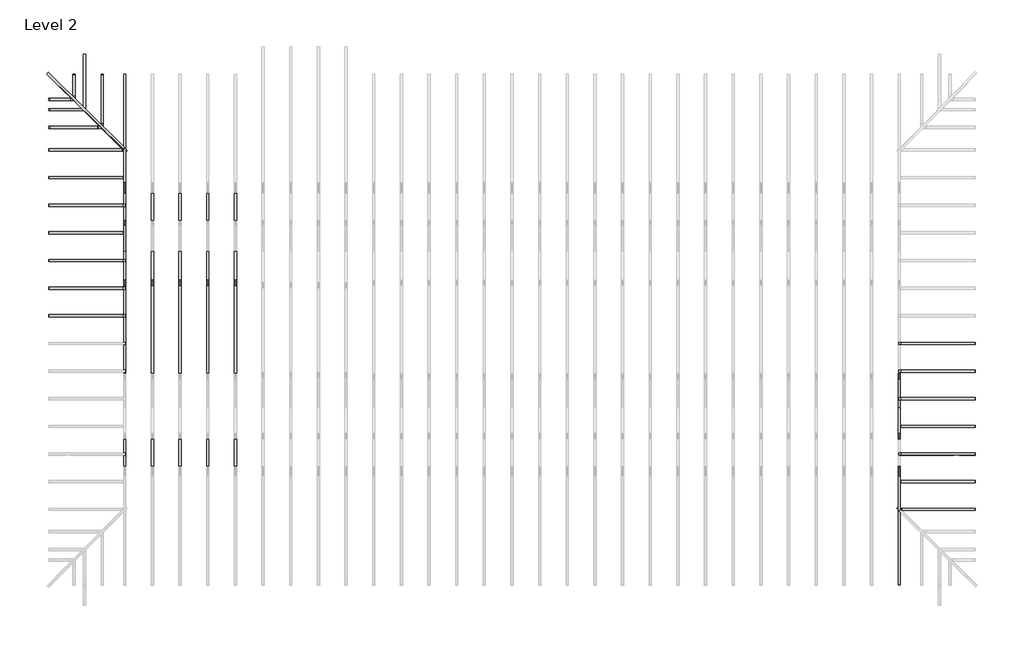
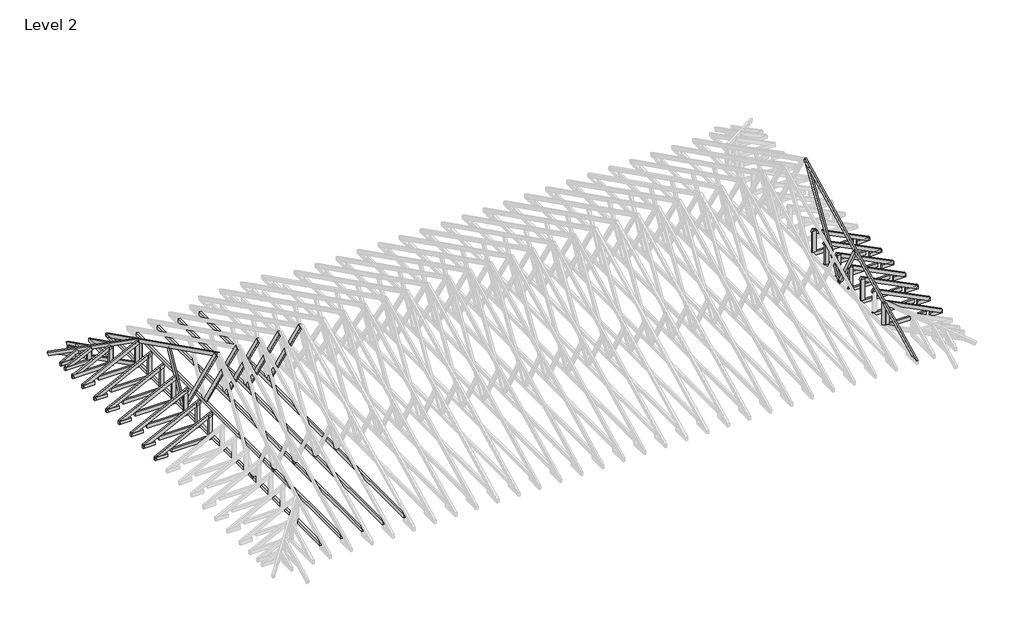
# One storey, part 3 of 5: 93 beams.
"""IFC4 building model written with IfcOpenShell, lengths in millimetres."""

import ifcopenshell
import ifcopenshell.guid

model = None  # the IFC model being written
_history = None  # IfcOwnerHistory: only IFC2X3 demands one
_inside = {}  # id of a spatial element -> (the spatial element, [elements in it])
_under = {}  # id of a project, library or spatial element -> (it, [spatial elements below it])
_declared = {}  # id of a project -> (the project, [libraries it declares])
_typed = {}  # id of a type object -> (the type object, [elements of that type])
_made_of = {}  # id of a material, layer set ... -> (it, [elements and type objects made of it])


def new_model(schema):
    """Start an empty IFC model of exactly this schema.

    Asked for "IFC4X3", IfcOpenShell would pick the latest addendum, in which some entities
    have other attributes; the version numbers below select the first issue.
    IFC2X3 requires an IfcOwnerHistory on every rooted entity: one is made here for all.
    """
    global model, _history
    if schema == "IFC4X3":
        model = ifcopenshell.file(schema_version=(4, 3, 0, 0))
    else:
        model = ifcopenshell.file(schema=schema)
    _inside.clear()
    _under.clear()
    _declared.clear()
    _typed.clear()
    _made_of.clear()
    _history = None
    if model.schema == "IFC2X3":
        org = make("IfcOrganization", Name="unknown")
        user = make(
            "IfcPersonAndOrganization",
            ThePerson=make("IfcPerson", FamilyName="unknown"),
            TheOrganization=org,
        )
        app = make(
            "IfcApplication",
            ApplicationDeveloper=org,
            Version="unknown",
            ApplicationFullName="unknown",
            ApplicationIdentifier="unknown",
        )
        _history = make(
            "IfcOwnerHistory",
            OwningUser=user,
            OwningApplication=app,
            ChangeAction="ADDED",
            CreationDate=0,
        )
    return model


def make(cls, **values):
    """One entity of the class cls with the attributes given. An attribute that is None is left unset."""
    return model.create_entity(
        cls, **{name: value for name, value in values.items() if value is not None}
    )


def rooted(cls, **values):
    """An entity with a GlobalId (a new one), such as an element, a storey or a relation."""
    return make(cls, GlobalId=ifcopenshell.guid.new(), OwnerHistory=_history, **values)


def si_unit(unit_type, name, prefix=None):
    """IfcSIUnit, for example si_unit("LENGTHUNIT", "METRE", prefix="MILLI")."""
    return make("IfcSIUnit", UnitType=unit_type, Prefix=prefix, Name=name)


def assignment(units):
    """IfcUnitAssignment: the units of a project."""
    return None if units is None else make("IfcUnitAssignment", Units=units)


def point(xyz):
    """IfcCartesianPoint."""
    return None if xyz is None else make("IfcCartesianPoint", Coordinates=xyz)


def direction(xyz):
    """IfcDirection."""
    return None if xyz is None else make("IfcDirection", DirectionRatios=xyz)


def frame(location, z_axis=None, x_axis=None):
    """IfcAxis2Placement3D, a coordinate frame: its origin and axes. An axis left out is left unset."""
    return make(
        "IfcAxis2Placement3D",
        Location=point(location),
        Axis=direction(z_axis),
        RefDirection=direction(x_axis),
    )


def origin():
    """The frame at (0, 0, 0) with its axes left unset."""
    return frame((0.0, 0.0, 0.0))


def place(relative_to, where):
    """IfcLocalPlacement: puts the frame where relative to a parent placement (None: the world)."""
    return make(
        "IfcLocalPlacement", PlacementRelTo=relative_to, RelativePlacement=where
    )


def context(
    kind, dimensions, precision=None, world=None, true_north=None, identifier=None
):
    """IfcGeometricRepresentationContext, for example the 3D "Model" context."""
    return make(
        "IfcGeometricRepresentationContext",
        ContextIdentifier=identifier,
        ContextType=kind,
        CoordinateSpaceDimension=dimensions,
        Precision=precision,
        WorldCoordinateSystem=world,
        TrueNorth=true_north,
    )


def project(units=None, contexts=None):
    """IfcProject with its units and contexts."""
    return rooted(
        "IfcProject",
        Name="project",
        RepresentationContexts=contexts,
        UnitsInContext=assignment(units),
    )


def spatial(cls, under=None, at=None, **own):
    """A site, building, storey or space (cls), placed at a placement, below another one or the project."""
    s = rooted(cls, ObjectPlacement=at, **own)
    if under is not None:
        _under.setdefault(under.id(), (under, []))[1].append(s)
    return s


def polyline(points):
    """IfcPolyline through the points."""
    return make("IfcPolyline", Points=[point(p) for p in points])


def outline(outer, holes=None, kind="AREA"):
    """IfcArbitraryClosedProfileDef: a profile drawn as a closed curve; with holes, ...WithVoids."""
    if holes is None:
        return make("IfcArbitraryClosedProfileDef", ProfileType=kind, OuterCurve=outer)
    return make(
        "IfcArbitraryProfileDefWithVoids",
        ProfileType=kind,
        OuterCurve=outer,
        InnerCurves=holes,
    )


def extrude(swept, where, along, depth):
    """IfcExtrudedAreaSolid: the profile swept, set in the frame where, extruded along a direction by depth."""
    return make(
        "IfcExtrudedAreaSolid",
        SweptArea=swept,
        Position=where,
        ExtrudedDirection=direction(along),
        Depth=depth,
    )


def shape(context_of_items, identifier, shape_type, items):
    """IfcShapeRepresentation: the items that make up one representation, for example the "Body"."""
    return make(
        "IfcShapeRepresentation",
        ContextOfItems=context_of_items,
        RepresentationIdentifier=identifier,
        RepresentationType=shape_type,
        Items=items,
    )


def source(mapping_origin, context_of_items, identifier, shape_type, items):
    """IfcRepresentationMap: a shape defined once, which mapped items show again and again."""
    return make(
        "IfcRepresentationMap",
        MappingOrigin=mapping_origin,
        MappedRepresentation=shape(context_of_items, identifier, shape_type, items),
    )


def transform(
    local_origin,
    x_axis=None,
    y_axis=None,
    z_axis=None,
    scale=None,
    scale2=None,
    scale3=None,
    uniform=True,
):
    """IfcCartesianTransformationOperator3D, or its non-uniform kind. x_axis, y_axis, z_axis: its Axis1, 2, 3."""
    if uniform:
        return make(
            "IfcCartesianTransformationOperator3D",
            Axis1=direction(x_axis),
            Axis2=direction(y_axis),
            LocalOrigin=point(local_origin),
            Scale=scale,
            Axis3=direction(z_axis),
        )
    return make(
        "IfcCartesianTransformationOperator3DnonUniform",
        Axis1=direction(x_axis),
        Axis2=direction(y_axis),
        LocalOrigin=point(local_origin),
        Scale=scale,
        Axis3=direction(z_axis),
        Scale2=scale2,
        Scale3=scale3,
    )


def mapped(mapping_source, mapping_target):
    """IfcMappedItem: shows the shape of a source again, moved by a transform."""
    return make(
        "IfcMappedItem", MappingSource=mapping_source, MappingTarget=mapping_target
    )


def made_of(thing, what):
    """Note that an element or type object is made of a material, layer set ...; save() writes the relation."""
    if what is not None:
        _made_of.setdefault(what.id(), (what, []))[1].append(thing)
    return thing


def element(
    cls,
    number,
    at=None,
    inside=None,
    cuts=None,
    type_object=None,
    material=None,
    context=None,
    identifier="Body",
    shape_type=None,
    held_by="IfcProductDefinitionShape",
    body=None,
    shapes=None,
    **own,
):
    """One element of the class cls, such as IfcWall. Its Tag is "e" and its number.

    at: its placement. inside: the storey or other place that contains it. cuts: it is an
    opening in that element (IfcRelVoidsElement). A single representation is given by context,
    identifier, shape_type and body (its items); several are given by shapes. held_by: the class
    of the entity that holds the representations. save() writes the other relations.
    """
    e = rooted(cls, Tag="e%d" % number, ObjectPlacement=at, **own)
    if body is not None:
        shapes = [shape(context, identifier, shape_type, body)]
    if shapes is not None:
        e.Representation = make(held_by, Representations=shapes)
    if inside is not None:
        _inside.setdefault(inside.id(), (inside, []))[1].append(e)
    if cuts is not None:
        rooted(
            "IfcRelVoidsElement", RelatingBuildingElement=cuts, RelatedOpeningElement=e
        )
    if type_object is not None:
        _typed.setdefault(type_object.id(), (type_object, []))[1].append(e)
    return made_of(e, material)


def aggregate(whole, parts):
    """IfcRelAggregates: a whole, such as a stair, and the parts it consists of."""
    return rooted("IfcRelAggregates", RelatingObject=whole, RelatedObjects=parts)


def save(model, path):
    """Write the relations noted so far, then the file.

    IfcRelAggregates (storeys below a building ...), IfcRelContainedInSpatialStructure (elements
    in a storey), IfcRelDefinesByType, IfcRelAssociatesMaterial and IfcRelDeclares: one each for
    every whole, place, type object, material and project.
    """
    for whole, parts in _under.values():
        aggregate(whole, parts)
    for where, things in _inside.values():
        rooted(
            "IfcRelContainedInSpatialStructure",
            RelatedElements=things,
            RelatingStructure=where,
        )
    for kind, things in _typed.values():
        rooted("IfcRelDefinesByType", RelatedObjects=things, RelatingType=kind)
    for what, things in _made_of.values():
        rooted("IfcRelAssociatesMaterial", RelatedObjects=things, RelatingMaterial=what)
    for by, libraries in _declared.values():
        rooted("IfcRelDeclares", RelatingContext=by, RelatedDefinitions=libraries)
    model.write(path)


def beam_90e8f76c(model_context):
    return source(origin(), model_context, "Body", "SweptSolid", [
        extrude(outline(polyline([(307.975, 25.4), (307.975, -25.4), (-47.625, -25.4), (-47.625, 25.4), (307.975, 25.4)])), frame((0.0, 0.0, -50.8), z_axis=(0.0, 0.0, 1.0), x_axis=(1.0, 0.0, 0.0)), (0.0, 0.0, 1.0), 101.6),
    ])


def beam_38027485(model_context):
    return source(origin(), model_context, "Body", "SweptSolid", [
        extrude(outline(polyline([(595.8662636, 25.4), (595.8662636, -25.4), (-609.6, -25.4), (-609.6, 25.4), (595.8662636, 25.4)])), frame((0.0, 0.0, -50.8), z_axis=(0.0, 0.0, 1.0), x_axis=(1.0, 0.0, 0.0)), (0.0, 0.0, 1.0), 101.6),
    ])


def beam_7745fe0f(model_context):
    return source(origin(), model_context, "Body", "SweptSolid", [
        extrude(outline(polyline([(393.7, 25.4), (393.7, -25.4), (-393.7, -25.4), (-393.7, 25.4), (393.7, 25.4)])), frame((0.0, 0.0, -50.8), z_axis=(0.0, 0.0, 1.0), x_axis=(1.0, 0.0, 0.0)), (0.0, 0.0, 1.0), 101.6),
    ])


def beam_85682148(model_context):
    return source(origin(), model_context, "Body", "SweptSolid", [
        extrude(outline(polyline([(595.8662636, -25.4), (-609.6, -25.4), (-609.6, 25.4), (595.8662636, 25.4), (595.8662636, -25.4)])), frame((0.0, 0.0, -50.8), z_axis=(0.0, 0.0, 1.0), x_axis=(1.0, 0.0, 0.0)), (0.0, 0.0, 1.0), 101.6),
    ])


def beam_154fe962(model_context):
    return source(origin(), model_context, "Body", "SweptSolid", [
        extrude(outline(polyline([(228.5999994, 25.4), (228.5999994, -25.4), (-228.6, -25.4), (-228.6, 25.4), (228.5999994, 25.4)])), frame((0.0, 0.0, -50.8), z_axis=(0.0, 0.0, 1.0), x_axis=(1.0, 0.0, 0.0)), (0.0, 0.0, 1.0), 101.6),
    ])


def beam_90eea034(model_context):
    return source(origin(), model_context, "Body", "SweptSolid", [
        extrude(outline(polyline([(821.193698, 25.4), (821.193698, -25.4), (-819.5010489, -25.4), (-819.5010489, 25.4), (821.193698, 25.4)])), frame((0.0, 0.0, -50.8), z_axis=(0.0, 0.0, 1.0), x_axis=(1.0, 0.0, 0.0)), (0.0, 0.0, 1.0), 101.6),
    ])


def beam_a4242642(model_context):
    return source(origin(), model_context, "Body", "SweptSolid", [
        extrude(outline(polyline([(5145.3336481, 25.4), (5145.3336481, -25.4), (-5145.3336481, -25.4), (-5145.3336481, 25.4), (5145.3336481, 25.4)])), frame((0.0, 0.0, -50.8), z_axis=(0.0, 0.0, 1.0), x_axis=(1.0, 0.0, 0.0)), (0.0, 0.0, 1.0), 101.6),
    ])


def beam_16181373(model_context):
    return source(origin(), model_context, "Body", "SweptSolid", [
        extrude(outline(polyline([(819.5010489, 25.4), (819.5010489, -25.4), (-821.193698, -25.4), (-821.193698, 25.4), (819.5010489, 25.4)])), frame((0.0, 0.0, -50.8), z_axis=(0.0, 0.0, 1.0), x_axis=(1.0, 0.0, 0.0)), (0.0, 0.0, 1.0), 101.6),
    ])


def beam_fc8bf4ae(model_context):
    return source(origin(), model_context, "Body", "SweptSolid", [
        extrude(outline(polyline([(1562.6646551, 25.4), (1562.6646551, -25.4), (-1550.1468127, -25.4), (-1550.1468127, 25.4), (1562.6646551, 25.4)])), frame((0.0, 0.0, -50.8), z_axis=(0.0, 0.0, 1.0), x_axis=(1.0, 0.0, 0.0)), (0.0, 0.0, 1.0), 101.6),
    ])


def beam_e838d316(model_context):
    return source(origin(), model_context, "Body", "SweptSolid", [
        extrude(outline(polyline([(1561.1045551, 25.4), (1561.1045551, -25.4), (-1572.5300502, -25.4), (-1572.5300502, 25.4), (1561.1045551, 25.4)])), frame((0.0, 0.0, -50.8), z_axis=(0.0, 0.0, 1.0), x_axis=(1.0, 0.0, 0.0)), (0.0, 0.0, 1.0), 101.6),
    ])


def beam_9afb64f6(model_context):
    return source(origin(), model_context, "Body", "SweptSolid", [
        extrude(outline(polyline([(365.3019367, 25.4), (365.3019367, -25.4), (-314.5019367, -25.4), (-314.5019367, 25.4), (365.3019367, 25.4)])), frame((0.0, 0.0, -50.8), z_axis=(0.0, 0.0, 1.0), x_axis=(1.0, 0.0, 0.0)), (0.0, 0.0, 1.0), 101.6),
    ])


def beam_87710fdd(model_context):
    return source(origin(), model_context, "Body", "SweptSolid", [
        extrude(outline(polyline([(147.1272806, 25.4), (147.1272806, -25.4), (-142.875, -25.4), (-142.875, 25.4), (147.1272806, 25.4)])), frame((0.0, 0.0, -50.8), z_axis=(0.0, 0.0, 1.0), x_axis=(1.0, 0.0, 0.0)), (0.0, 0.0, 1.0), 101.6),
    ])


def beam_29c6d41d(model_context):
    return source(origin(), model_context, "Body", "SweptSolid", [
        extrude(outline(polyline([(350.5042173, 25.4), (350.5042173, -25.4), (-295.4519367, -25.4), (-295.4519367, 25.4), (350.5042173, 25.4)])), frame((0.0, 0.0, -50.8), z_axis=(0.0, 0.0, 1.0), x_axis=(1.0, 0.0, 0.0)), (0.0, 0.0, 1.0), 101.6),
    ])


def beam_af5d22dc(model_context):
    return source(origin(), model_context, "Body", "SweptSolid", [
        extrude(outline(polyline([(571.5, 25.4), (571.5, -25.4), (-609.6, -25.4), (-609.6, 25.4), (571.5, 25.4)])), frame((0.0, 0.0, -50.8), z_axis=(0.0, 0.0, 1.0), x_axis=(1.0, 0.0, 0.0)), (0.0, 0.0, 1.0), 101.6),
    ])


def beam_7b8fa6d1(model_context):
    return source(origin(), model_context, "Body", "SweptSolid", [
        extrude(outline(polyline([(270.7395597, 25.4), (270.7395597, -25.4), (-219.9395597, -25.4), (-219.9395597, 25.4), (270.7395597, 25.4)])), frame((0.0, 0.0, -50.8), z_axis=(0.0, 0.0, 1.0), x_axis=(1.0, 0.0, 0.0)), (0.0, 0.0, 1.0), 101.6),
    ])


def beam_5e172d94(model_context):
    return source(origin(), model_context, "Body", "SweptSolid", [
        extrude(outline(polyline([(595.8662636, 25.4), (595.8662636, -25.4), (-548.2789755, -25.4), (-548.2789755, 25.4), (595.8662636, 25.4)])), frame((0.0, 0.0, -50.8), z_axis=(0.0, 0.0, 1.0), x_axis=(1.0, 0.0, 0.0)), (0.0, 0.0, 1.0), 101.6),
    ])


def beam_42a29ae5(model_context):
    return source(origin(), model_context, "Body", "SweptSolid", [
        extrude(outline(polyline([(270.7395597, -25.4), (-219.9395597, -25.4), (-219.9395597, 25.4), (270.7395597, 25.4), (270.7395597, -25.4)])), frame((0.0, 0.0, -50.8), z_axis=(0.0, 0.0, 1.0), x_axis=(1.0, 0.0, 0.0)), (0.0, 0.0, 1.0), 101.6),
    ])


def beam_11c5b8ca(model_context):
    return source(origin(), model_context, "Body", "SweptSolid", [
        extrude(outline(polyline([(147.1272806, -25.4), (-142.875, -25.4), (-142.875, 25.4), (147.1272806, 25.4), (147.1272806, -25.4)])), frame((0.0, 0.0, -50.8), z_axis=(0.0, 0.0, 1.0), x_axis=(1.0, 0.0, 0.0)), (0.0, 0.0, 1.0), 101.6),
    ])


def beam_5ac0b85f(model_context):
    return source(origin(), model_context, "Body", "SweptSolid", [
        extrude(outline(polyline([(571.5, -25.4), (-584.2, -25.4), (-584.2, 25.4), (571.5, 25.4), (571.5, -25.4)])), frame((0.0, 0.0, -50.8), z_axis=(0.0, 0.0, 1.0), x_axis=(1.0, 0.0, 0.0)), (0.0, 0.0, 1.0), 101.6),
    ])


def beam_99e5442a(model_context):
    return source(origin(), model_context, "Body", "SweptSolid", [
        extrude(outline(polyline([(350.5042173, -25.4), (-295.4519367, -25.4), (-295.4519367, 25.4), (350.5042173, 25.4), (350.5042173, -25.4)])), frame((0.0, 0.0, -50.8), z_axis=(0.0, 0.0, 1.0), x_axis=(1.0, 0.0, 0.0)), (0.0, 0.0, 1.0), 101.6),
    ])


def beam_38e3f9e5(model_context):
    return source(origin(), model_context, "Body", "SweptSolid", [
        extrude(outline(polyline([(595.8662636, -25.4), (-548.2789755, -25.4), (-548.2789755, 25.4), (595.8662636, 25.4), (595.8662636, -25.4)])), frame((0.0, 0.0, -50.8), z_axis=(0.0, 0.0, 1.0), x_axis=(1.0, 0.0, 0.0)), (0.0, 0.0, 1.0), 101.6),
    ])


def beam_7aad778a(model_context):
    return source(origin(), model_context, "Body", "SweptSolid", [
        extrude(outline(polyline([(307.975, -25.4), (-47.625, -25.4), (-47.625, 25.4), (307.975, 25.4), (307.975, -25.4)])), frame((0.0, 0.0, -50.8), z_axis=(0.0, 0.0, 1.0), x_axis=(1.0, 0.0, 0.0)), (0.0, 0.0, 1.0), 101.6),
    ])


def beam_878446a4(model_context):
    return source(origin(), model_context, "Body", "SweptSolid", [
        extrude(outline(polyline([(63.8057136, 25.4), (63.8057136, -25.4), (-59.553433, -25.4), (-59.553433, 25.4), (63.8057136, 25.4)])), frame((0.0, 0.0, -50.8), z_axis=(0.0, 0.0, 1.0), x_axis=(1.0, 0.0, 0.0)), (0.0, 0.0, 1.0), 101.6),
    ])


def beam_bc99fd75(model_context):
    return source(origin(), model_context, "Body", "SweptSolid", [
        extrude(outline(polyline([(222.3387319, 25.4), (222.3387319, -25.4), (-231.775, -25.4), (-231.775, 25.4), (222.3387319, 25.4)])), frame((0.0, 0.0, -50.8), z_axis=(0.0, 0.0, 1.0), x_axis=(1.0, 0.0, 0.0)), (0.0, 0.0, 1.0), 101.6),
    ])


def beam_efe25585(model_context):
    return source(origin(), model_context, "Body", "SweptSolid", [
        extrude(outline(polyline([(222.3387319, -25.4), (-231.775, -25.4), (-231.775, 25.4), (222.3387319, 25.4), (222.3387319, -25.4)])), frame((0.0, 0.0, -50.8), z_axis=(0.0, 0.0, 1.0), x_axis=(1.0, 0.0, 0.0)), (0.0, 0.0, 1.0), 101.6),
    ])


def beam_dfed05dc(model_context):
    return source(origin(), model_context, "Body", "SweptSolid", [
        extrude(outline(polyline([(63.8057136, -25.4), (-59.553433, -25.4), (-59.553433, 25.4), (63.8057136, 25.4), (63.8057136, -25.4)])), frame((0.0, 0.0, -50.8), z_axis=(0.0, 0.0, 1.0), x_axis=(1.0, 0.0, 0.0)), (0.0, 0.0, 1.0), 101.6),
    ])


def beam_b8261971(model_context):
    return source(origin(), model_context, "Body", "SweptSolid", [
        extrude(outline(polyline([(233.4866591, 25.4), (233.4866591, -25.4), (-1841.8619641, -25.4), (-1841.8619641, 25.4), (233.4866591, 25.4)])), frame((0.0, 0.0, -50.8), z_axis=(0.0, 0.0, 1.0), x_axis=(1.0, 0.0, 0.0)), (0.0, 0.0, 1.0), 101.6),
    ])


def beam_925b2549(model_context):
    return source(origin(), model_context, "Body", "SweptSolid", [
        extrude(outline(polyline([(371.7582386, -25.4), (-368.3, -25.4), (-368.3, 25.4), (371.7582386, 25.4), (371.7582386, -25.4)])), frame((0.0, 0.0, -50.8), z_axis=(0.0, 0.0, 1.0), x_axis=(1.0, 0.0, 0.0)), (0.0, 0.0, 1.0), 101.6),
    ])


model = new_model("IFC4")

# Units and contexts
model_context = context("Model", 3, world=origin())
ifc_project = project(units=[si_unit("LENGTHUNIT", "METRE", prefix="MILLI")], contexts=[model_context])

# Site, building, storey
site = spatial("IfcSite", under=ifc_project)
building = spatial("IfcBuilding", under=site)
storey = spatial("IfcBuildingStorey", under=building, Name="Level 2", Elevation=2768.6)

# Beams
placement = place(None, origin())
element("IfcBeam", 1, ObjectType="Dimension Lumber : BLDG 6241 2X4\" TRUSS MEMBER", at=placement, inside=storey, context=model_context, shape_type="SweptSolid", body=[
    extrude(outline(polyline([(0.0, -50.8), (0.0, 0.0), (6302.2496334, 0.0), (6302.2496334, -50.8), (0.0, -50.8)])), frame((-16607.414829, -17.2791662, 5496.1115355), z_axis=(0.0, 0.447213595499958, 0.894427190999916), x_axis=(0.0, 0.894427190999916, -0.447213595499958)), (0.0, 0.0, 1.0), 101.6),
])
element("IfcBeam", 2, ObjectType="Dimension Lumber : BLDG 6241 2X4\" TRUSS MEMBER", at=placement, inside=storey, context=model_context, shape_type="SweptSolid", body=[
    extrude(outline(polyline([(0.0, -50.8), (0.0, 0.0), (1828.8, 0.0), (1828.8, -50.8), (0.0, -50.8)])), frame((-18206.2149687, 3404.3284114, 2681.1076769), z_axis=(-0.44721359549995937, 0.0, 0.8944271909999152), x_axis=(0.8944271909999152, 0.0, 0.44721359549995937)), (0.0, 0.0, 1.0), 101.6),
])
element("IfcBeam", 3, ObjectType="Dimension Lumber : BLDG 6241 2X4\" TRUSS MEMBER", at=placement, inside=storey, context=model_context, shape_type="SweptSolid", body=[
    extrude(outline(polyline([(1e-07, -50.8), (0.0, 0.0), (2518.7475141, 0.0), (2518.7475141, -50.8), (1e-07, -50.8)])), frame((-16592.3107327, 3976.1580779, 3516.9362486), z_axis=(-0.2218309319850432, 0.2532052771584921, 0.9416358772018717), x_axis=(-0.6716162760239249, 0.6604274920267121, -0.33580813801196385)), (0.0, 0.0, 1.0), 101.6),
])
element("IfcBeam", 4, ObjectType="Dimension Lumber : BLDG 6241 2X4\" TRUSS MEMBER", at=placement, inside=storey, context=model_context, shape_type="SweptSolid", body=[
    extrude(outline(polyline([(0.0, -50.8), (0.0, 0.0), (1203.6219076, 0.0), (1203.6219076, -50.8), (0.0, -50.8)])), frame((-18207.7449824, 4509.2284114, 2680.3426701), z_axis=(-0.44721359549995937, 0.0, 0.8944271909999152), x_axis=(0.8944271909999152, 0.0, 0.44721359549995937)), (0.0, 0.0, 1.0), 101.6),
])
element("IfcBeam", 5, ObjectType="Dimension Lumber : BLDG 6241 2X4\" TRUSS MEMBER", at=placement, inside=storey, context=model_context, shape_type="SweptSolid", body=[
    extrude(outline(polyline([(0.0, -50.8), (0.0, 0.0), (844.55, 0.0), (844.55, -50.8), (0.0, -50.8)])), frame((-18212.4885612, 4902.9284114, 2677.9708807), z_axis=(-0.4472135954999599, 0.0, 0.894427190999915), x_axis=(0.894427190999915, 0.0, 0.4472135954999599)), (0.0, 0.0, 1.0), 101.6),
])
element("IfcBeam", 6, ObjectType="Dimension Lumber : BLDG 6241 2X4\" TRUSS MEMBER", at=placement, inside=storey, context=model_context, shape_type="SweptSolid", body=[
    extrude(outline(polyline([(0.0, -50.8), (0.0, 0.0), (6302.3539791, 0.0), (6302.3539791, -50.8), (0.0, -50.8)])), frame((461.385171, -5565.5155384, 2678.5857718), z_axis=(0.0, -0.447213595499958, 0.894427190999916), x_axis=(0.0, 0.894427190999916, 0.447213595499958)), (0.0, 0.0, 1.0), 101.6),
])
element("IfcBeam", 7, ObjectType="Dimension Lumber : BLDG 6241 2X4\" TRUSS MEMBER", at=placement, inside=storey, context=model_context, shape_type="SweptSolid", body=[
    extrude(outline(polyline([(0.0, -50.8), (0.0, 0.0), (1787.5128974, 0.0), (1787.5128974, -50.8), (0.0, -50.8)])), frame((-18206.2149687, 4013.9284114, 2681.1076769), z_axis=(-0.44721359549995937, 0.0, 0.8944271909999152), x_axis=(0.8944271909999152, 0.0, 0.44721359549995937)), (0.0, 0.0, 1.0), 101.6),
])
element("IfcBeam", 8, ObjectType="Dimension Lumber : BLDG 6241 2X4\" TRUSS MEMBER", at=placement, inside=storey, context=model_context, shape_type="SweptSolid", body=[
    extrude(outline(polyline([(0.0, -50.8), (0.0, 0.0), (1828.8, 0.0), (1828.8, -50.8), (0.0, -50.8)])), frame((-18206.2149687, 2794.7284114, 2681.1076769), z_axis=(-0.44721359549995937, 0.0, 0.8944271909999152), x_axis=(0.8944271909999152, 0.0, 0.44721359549995937)), (0.0, 0.0, 1.0), 101.6),
])
element("IfcBeam", 9, ObjectType="Dimension Lumber : BLDG 6241 2X4\" TRUSS MEMBER", at=placement, inside=storey, context=model_context, shape_type="SweptSolid", body=[
    extrude(outline(polyline([(0.0, -50.8), (0.0, 0.0), (1828.8, 0.0), (1828.8, -50.8), (0.0, -50.8)])), frame((-18206.2149687, 2185.1284114, 2681.1076769), z_axis=(-0.44721359549995937, 0.0, 0.8944271909999152), x_axis=(0.8944271909999152, 0.0, 0.44721359549995937)), (0.0, 0.0, 1.0), 101.6),
])
element("IfcBeam", 10, ObjectType="Dimension Lumber : BLDG 6241 2X4\" TRUSS MEMBER", at=placement, inside=storey, context=model_context, shape_type="SweptSolid", body=[
    extrude(outline(polyline([(0.0, -50.8), (0.0, 0.0), (1828.8, 0.0), (1828.8, -50.8), (0.0, -50.8)])), frame((-18206.2149687, 1575.5284114, 2681.1076769), z_axis=(-0.44721359549995937, 0.0, 0.8944271909999152), x_axis=(0.8944271909999152, 0.0, 0.44721359549995937)), (0.0, 0.0, 1.0), 101.6),
])
element("IfcBeam", 11, ObjectType="Dimension Lumber : BLDG 6241 2X4\" TRUSS MEMBER", at=placement, inside=storey, context=model_context, shape_type="SweptSolid", body=[
    extrude(outline(polyline([(0.0, -50.8), (0.0, 0.0), (1828.8, 0.0), (1828.8, -50.8), (0.0, -50.8)])), frame((-18206.2149687, 965.9284114, 2681.1076769), z_axis=(-0.44721359549995937, 0.0, 0.8944271909999152), x_axis=(0.8944271909999152, 0.0, 0.44721359549995937)), (0.0, 0.0, 1.0), 101.6),
])
element("IfcBeam", 12, ObjectType="Dimension Lumber : BLDG 6241 2X4\" TRUSS MEMBER", at=placement, inside=storey, context=model_context, shape_type="SweptSolid", body=[
    extrude(outline(polyline([(0.0, -50.8), (0.0, 0.0), (1828.8, 0.0), (1828.8, -50.8), (0.0, -50.8)])), frame((-18206.2149687, 356.3284114, 2681.1076769), z_axis=(-0.44721359549995937, 0.0, 0.8944271909999152), x_axis=(0.8944271909999152, 0.0, 0.44721359549995937)), (0.0, 0.0, 1.0), 101.6),
])
element("IfcBeam", 13, ObjectType="Dimension Lumber : BLDG 6241 2X4\" TRUSS MEMBER", at=placement, inside=storey, context=model_context, shape_type="SweptSolid", body=[
    extrude(outline(polyline([(0.0, 50.8), (1203.6219076, 50.8), (1203.6219076, 0.0), (0.0, 0.0), (0.0, 50.8)])), frame((-17102.714829, 5614.2585647, 2680.3426701), z_axis=(0.0, 0.44721359549995937, 0.8944271909999152), x_axis=(0.0, -0.8944271909999152, 0.44721359549995937)), (0.0, 0.0, 1.0), 101.6),
])
element("IfcBeam", 14, ObjectType="Dimension Lumber : BLDG 6241 2X4\" TRUSS MEMBER", at=placement, inside=storey, context=model_context, shape_type="SweptSolid", body=[
    extrude(outline(polyline([(0.0, 50.8), (1334.5727744, 50.8), (1334.5727744, 0.0), (0.0, 0.0), (0.0, 50.8)])), frame((-17496.414829, 6057.2918371, 2458.8260339), z_axis=(0.0, 0.4472135954999599, 0.894427190999915), x_axis=(0.0, -0.894427190999915, 0.4472135954999599)), (0.0, 0.0, 1.0), 101.6),
])
element("IfcBeam", 15, ObjectType="Dimension Lumber : BLDG 6241 2X4\" TRUSS MEMBER", at=placement, inside=storey, context=model_context, shape_type="SweptSolid", body=[
    extrude(outline(polyline([(0.0, 50.8), (1828.8, 50.8), (1828.8, 0.0), (0.0, 0.0), (0.0, 50.8)])), frame((2110.9853106, -253.2715886, 2681.1076769), z_axis=(0.44721359549995937, 0.0, 0.8944271909999152), x_axis=(-0.8944271909999152, 0.0, 0.44721359549995937)), (0.0, 0.0, 1.0), 101.6),
])
element("IfcBeam", 16, ObjectType="Dimension Lumber : BLDG 6241 2X4\" TRUSS MEMBER", at=placement, inside=storey, context=model_context, shape_type="SweptSolid", body=[
    extrude(outline(polyline([(0.0, 50.8), (1828.8, 50.8), (1828.8, 0.0), (0.0, 0.0), (0.0, 50.8)])), frame((2110.9853106, -862.8715886, 2681.1076769), z_axis=(0.44721359549995937, 0.0, 0.8944271909999152), x_axis=(-0.8944271909999152, 0.0, 0.44721359549995937)), (0.0, 0.0, 1.0), 101.6),
])
element("IfcBeam", 17, ObjectType="Dimension Lumber : BLDG 6241 2X4\" TRUSS MEMBER", at=placement, inside=storey, context=model_context, shape_type="SweptSolid", body=[
    extrude(outline(polyline([(0.0, 50.8), (1828.8, 50.8), (1828.8, 0.0), (0.0, 0.0), (0.0, 50.8)])), frame((2110.9853106, -1472.4715886, 2681.1076769), z_axis=(0.44721359549995937, 0.0, 0.8944271909999152), x_axis=(-0.8944271909999152, 0.0, 0.44721359549995937)), (0.0, 0.0, 1.0), 101.6),
])
element("IfcBeam", 18, ObjectType="Dimension Lumber : BLDG 6241 2X4\" TRUSS MEMBER", at=placement, inside=storey, context=model_context, shape_type="SweptSolid", body=[
    extrude(outline(polyline([(0.0, 50.8), (1828.8, 50.8), (1828.8, 0.0), (0.0, 0.0), (0.0, 50.8)])), frame((2110.9853106, -2082.0715886, 2681.1076769), z_axis=(0.44721359549995937, 0.0, 0.8944271909999152), x_axis=(-0.8944271909999152, 0.0, 0.44721359549995937)), (0.0, 0.0, 1.0), 101.6),
])
element("IfcBeam", 19, ObjectType="Dimension Lumber : BLDG 6241 2X4\" TRUSS MEMBER", at=placement, inside=storey, context=model_context, shape_type="SweptSolid", body=[
    extrude(outline(polyline([(0.0, 50.8), (1828.8, 50.8), (1828.8, 0.0), (0.0, 0.0), (0.0, 50.8)])), frame((2110.9853106, -2691.6715886, 2681.1076769), z_axis=(0.44721359549995937, 0.0, 0.8944271909999152), x_axis=(-0.8944271909999152, 0.0, 0.44721359549995937)), (0.0, 0.0, 1.0), 101.6),
])
element("IfcBeam", 20, ObjectType="Dimension Lumber : BLDG 6241 2X4\" TRUSS MEMBER", at=placement, inside=storey, context=model_context, shape_type="SweptSolid", body=[
    extrude(outline(polyline([(0.0, 50.8), (1828.8, 50.8), (1828.8, 0.0), (0.0, 0.0), (0.0, 50.8)])), frame((2110.9853106, -3301.2715886, 2681.1076769), z_axis=(0.44721359549995937, 0.0, 0.8944271909999152), x_axis=(-0.8944271909999152, 0.0, 0.44721359549995937)), (0.0, 0.0, 1.0), 101.6),
])
element("IfcBeam", 21, ObjectType="Dimension Lumber : BLDG 6241 2X4\" TRUSS MEMBER", at=placement, inside=storey, context=model_context, shape_type="SweptSolid", body=[
    extrude(outline(polyline([(0.0, 50.8), (1787.5128973, 50.8), (1787.5128973, 0.0), (0.0, 0.0), (0.0, 50.8)])), frame((2110.9853106, -3910.8715886, 2681.1076769), z_axis=(0.44721359549995937, 0.0, 0.8944271909999152), x_axis=(-0.8944271909999152, 0.0, 0.44721359549995937)), (0.0, 0.0, 1.0), 101.6),
])
element("IfcBeam", 22, ObjectType="Dimension Lumber : BLDG 6241 2X4\" TRUSS MEMBER", at=placement, inside=storey, context=model_context, shape_type="SweptSolid", body=[
    extrude(outline(polyline([(0.0, -50.8), (0.0, 0.0), (546.1, 0.0), (546.1, -50.8), (0.0, -50.8)])), frame((-18212.1757804, 5131.5284114, 2678.127271), z_axis=(-0.4472135954999593, 0.0, 0.8944271909999153), x_axis=(0.8944271909999153, 0.0, 0.4472135954999593)), (0.0, 0.0, 1.0), 101.6),
])
element("IfcBeam", 23, ObjectType="Dimension Lumber : BLDG 6241 2X4\" TRUSS MEMBER", at=placement, inside=storey, context=model_context, shape_type="SweptSolid", body=[
    extrude(outline(polyline([(0.0, 50.8), (546.1, 50.8), (546.1, 0.0), (0.0, 0.0), (0.0, 50.8)])), frame((-17725.014829, 5618.6893628, 2678.127271), z_axis=(0.0, 0.4472135954999592, 0.8944271909999153), x_axis=(0.0, -0.8944271909999153, 0.4472135954999592)), (0.0, 0.0, 1.0), 101.6),
])
beam_shape = beam_90e8f76c(model_context)
element("IfcBeam", 24, ObjectType="Dimension Lumber : BLDG 6241 2X4\" TRUSS MEMBER", at=placement, inside=storey, context=model_context, shape_type="MappedRepresentation", body=[
    mapped(beam_shape, transform((-18210.789829, 3378.9284114, 2717.8), x_axis=(1.0, 0.0, 0.0), y_axis=(0.0, 1.0, 0.0), z_axis=(0.0, 0.0, 1.0))),
])
element("IfcBeam", 25, ObjectType="Dimension Lumber : BLDG 6241 2X4\" TRUSS MEMBER", at=placement, inside=storey, context=model_context, shape_type="MappedRepresentation", body=[
    mapped(beam_shape, transform((-18210.789829, 3988.5284114, 2717.8), x_axis=(1.0, 0.0, 0.0), y_axis=(0.0, 1.0, 0.0), z_axis=(0.0, 0.0, 1.0))),
])
element("IfcBeam", 26, ObjectType="Dimension Lumber : BLDG 6241 2X4\" TRUSS MEMBER", at=placement, inside=storey, context=model_context, shape_type="MappedRepresentation", body=[
    mapped(beam_shape, transform((-18210.789829, 2769.3284114, 2717.8), x_axis=(1.0, 0.0, 0.0), y_axis=(0.0, 1.0, 0.0), z_axis=(0.0, 0.0, 1.0))),
])
element("IfcBeam", 27, ObjectType="Dimension Lumber : BLDG 6241 2X4\" TRUSS MEMBER", at=placement, inside=storey, context=model_context, shape_type="MappedRepresentation", body=[
    mapped(beam_shape, transform((-18210.789829, 2159.7284114, 2717.8), x_axis=(1.0, 0.0, 0.0), y_axis=(0.0, 1.0, 0.0), z_axis=(0.0, 0.0, 1.0))),
])
element("IfcBeam", 28, ObjectType="Dimension Lumber : BLDG 6241 2X4\" TRUSS MEMBER", at=placement, inside=storey, context=model_context, shape_type="MappedRepresentation", body=[
    mapped(beam_shape, transform((-18210.789829, 1550.1284114, 2717.8), x_axis=(1.0, 0.0, 0.0), y_axis=(0.0, 1.0, 0.0), z_axis=(0.0, 0.0, 1.0))),
])
element("IfcBeam", 29, ObjectType="Dimension Lumber : BLDG 6241 2X4\" TRUSS MEMBER", at=placement, inside=storey, context=model_context, shape_type="MappedRepresentation", body=[
    mapped(beam_shape, transform((-18210.789829, 940.5284114, 2717.8), x_axis=(1.0, 0.0, 0.0), y_axis=(0.0, 1.0, 0.0), z_axis=(0.0, 0.0, 1.0))),
])
element("IfcBeam", 30, ObjectType="Dimension Lumber : BLDG 6241 2X4\" TRUSS MEMBER", at=placement, inside=storey, context=model_context, shape_type="MappedRepresentation", body=[
    mapped(beam_shape, transform((-18210.789829, 330.9284114, 2717.8), x_axis=(1.0, 0.0, 0.0), y_axis=(0.0, 1.0, 0.0), z_axis=(0.0, 0.0, 1.0))),
])
beam_2_shape = beam_38027485(model_context)
element("IfcBeam", 31, ObjectType="Dimension Lumber : BLDG 6241 2X4\" TRUSS MEMBER", at=placement, inside=storey, context=model_context, shape_type="MappedRepresentation", body=[
    mapped(beam_2_shape, transform((-17191.614829, 3378.9284114, 2819.4), x_axis=(-1.0, 0.0, 0.0), y_axis=(0.0, -1.0, 0.0), z_axis=(0.0, 0.0, 1.0))),
])
element("IfcBeam", 32, ObjectType="Dimension Lumber : BLDG 6241 2X4\" TRUSS MEMBER", at=placement, inside=storey, context=model_context, shape_type="MappedRepresentation", body=[
    mapped(beam_2_shape, transform((-17191.614829, 2769.3284114, 2819.4), x_axis=(-1.0, 0.0, 0.0), y_axis=(0.0, -1.0, 0.0), z_axis=(0.0, 0.0, 1.0))),
])
element("IfcBeam", 33, ObjectType="Dimension Lumber : BLDG 6241 2X4\" TRUSS MEMBER", at=placement, inside=storey, context=model_context, shape_type="MappedRepresentation", body=[
    mapped(beam_2_shape, transform((-17191.614829, 2159.7284114, 2819.4), x_axis=(-1.0, 0.0, 0.0), y_axis=(0.0, -1.0, 0.0), z_axis=(0.0, 0.0, 1.0))),
])
element("IfcBeam", 34, ObjectType="Dimension Lumber : BLDG 6241 2X4\" TRUSS MEMBER", at=placement, inside=storey, context=model_context, shape_type="MappedRepresentation", body=[
    mapped(beam_2_shape, transform((-17191.614829, 1550.1284114, 2819.4), x_axis=(-1.0, 0.0, 0.0), y_axis=(0.0, -1.0, 0.0), z_axis=(0.0, 0.0, 1.0))),
])
element("IfcBeam", 35, ObjectType="Dimension Lumber : BLDG 6241 2X4\" TRUSS MEMBER", at=placement, inside=storey, context=model_context, shape_type="MappedRepresentation", body=[
    mapped(beam_2_shape, transform((-17191.614829, 940.5284114, 2819.4), x_axis=(-1.0, 0.0, 0.0), y_axis=(0.0, -1.0, 0.0), z_axis=(0.0, 0.0, 1.0))),
])
element("IfcBeam", 36, ObjectType="Dimension Lumber : BLDG 6241 2X4\" TRUSS MEMBER", at=placement, inside=storey, context=model_context, shape_type="MappedRepresentation", body=[
    mapped(beam_2_shape, transform((-17191.614829, 330.9284114, 2819.4), x_axis=(-1.0, 0.0, 0.0), y_axis=(0.0, -1.0, 0.0), z_axis=(0.0, 0.0, 1.0))),
])
beam_3_shape = beam_7745fe0f(model_context)
element("IfcBeam", 37, ObjectType="Dimension Lumber : BLDG 6241 2X4\" TRUSS MEMBER", at=placement, inside=storey, context=model_context, shape_type="MappedRepresentation", body=[
    mapped(beam_3_shape, transform((-17864.714829, 4877.5284114, 2728.7708807), x_axis=(-1.0, 0.0, 0.0), y_axis=(0.0, -1.0, 0.0), z_axis=(0.0, 0.0, 1.0))),
])
beam_4_shape = beam_85682148(model_context)
element("IfcBeam", 38, ObjectType="Dimension Lumber : BLDG 6241 2X4\" TRUSS MEMBER", at=placement, inside=storey, context=model_context, shape_type="MappedRepresentation", body=[
    mapped(beam_4_shape, transform((1096.385171, -278.6715886, 2819.4), x_axis=(1.0, 0.0, 0.0), y_axis=(0.0, 1.0, 0.0), z_axis=(0.0, 0.0, 1.0))),
])
element("IfcBeam", 39, ObjectType="Dimension Lumber : BLDG 6241 2X4\" TRUSS MEMBER", at=placement, inside=storey, context=model_context, shape_type="MappedRepresentation", body=[
    mapped(beam_4_shape, transform((1096.385171, -888.2715886, 2819.4), x_axis=(1.0, 0.0, 0.0), y_axis=(0.0, 1.0, 0.0), z_axis=(0.0, 0.0, 1.0))),
])
element("IfcBeam", 40, ObjectType="Dimension Lumber : BLDG 6241 2X4\" TRUSS MEMBER", at=placement, inside=storey, context=model_context, shape_type="MappedRepresentation", body=[
    mapped(beam_4_shape, transform((1096.385171, -1497.8715886, 2819.4), x_axis=(1.0, 0.0, 0.0), y_axis=(0.0, 1.0, 0.0), z_axis=(0.0, 0.0, 1.0))),
])
element("IfcBeam", 41, ObjectType="Dimension Lumber : BLDG 6241 2X4\" TRUSS MEMBER", at=placement, inside=storey, context=model_context, shape_type="MappedRepresentation", body=[
    mapped(beam_4_shape, transform((1096.385171, -2107.4715886, 2819.4), x_axis=(1.0, 0.0, 0.0), y_axis=(0.0, 1.0, 0.0), z_axis=(0.0, 0.0, 1.0))),
])
element("IfcBeam", 42, ObjectType="Dimension Lumber : BLDG 6241 2X4\" TRUSS MEMBER", at=placement, inside=storey, context=model_context, shape_type="MappedRepresentation", body=[
    mapped(beam_4_shape, transform((1096.385171, -2717.0715886, 2819.4), x_axis=(1.0, 0.0, 0.0), y_axis=(0.0, 1.0, 0.0), z_axis=(0.0, 0.0, 1.0))),
])
element("IfcBeam", 43, ObjectType="Dimension Lumber : BLDG 6241 2X4\" TRUSS MEMBER", at=placement, inside=storey, context=model_context, shape_type="MappedRepresentation", body=[
    mapped(beam_4_shape, transform((1096.385171, -3326.6715886, 2819.4), x_axis=(1.0, 0.0, 0.0), y_axis=(0.0, 1.0, 0.0), z_axis=(0.0, 0.0, 1.0))),
])
beam_5_shape = beam_154fe962(model_context)
element("IfcBeam", 44, ObjectType="Dimension Lumber : BLDG 6241 2X4\" TRUSS MEMBER", at=placement, inside=storey, context=model_context, shape_type="MappedRepresentation", body=[
    mapped(beam_5_shape, transform((-16582.014829, 5436.3284114, 2717.8), x_axis=(0.0, -1.0, 0.0), y_axis=(1.0, 0.0, 0.0), z_axis=(0.0, 0.0, 1.0))),
])
beam_6_shape = beam_90eea034(model_context)
element("IfcBeam", 45, ObjectType="Dimension Lumber : BLDG 6241 2X4\" TRUSS MEMBER", at=placement, inside=storey, context=model_context, shape_type="MappedRepresentation", body=[
    mapped(beam_6_shape, transform((-16582.014829, 2147.8781861, 3552.5770493), x_axis=(0.0, -0.4803172630852001, -0.8770948220017848), y_axis=(-1.0, 0.0, 0.0), z_axis=(0.0, 0.8770948220017848, -0.4803172630852001))),
])
beam_7_shape = beam_a4242642(model_context)
element("IfcBeam", 46, ObjectType="Dimension Lumber : BLDG 6241 2X4\" TRUSS MEMBER", at=placement, inside=storey, context=model_context, shape_type="MappedRepresentation", body=[
    mapped(beam_7_shape, transform((-16582.014829, 26.1284114, 2819.4), x_axis=(0.0, -1.0, 0.0), y_axis=(1.0, 0.0, 0.0), z_axis=(0.0, 0.0, 1.0))),
])
element("IfcBeam", 47, ObjectType="Dimension Lumber : BLDG 6241 2X4\" TRUSS MEMBER", at=placement, inside=storey, context=model_context, shape_type="MappedRepresentation", body=[
    mapped(beam_7_shape, transform((-15972.414829, 26.1284114, 2819.4), x_axis=(0.0, -1.0, 0.0), y_axis=(1.0, 0.0, 0.0), z_axis=(0.0, 0.0, 1.0))),
])
element("IfcBeam", 48, ObjectType="Dimension Lumber : BLDG 6241 2X4\" TRUSS MEMBER", at=placement, inside=storey, context=model_context, shape_type="MappedRepresentation", body=[
    mapped(beam_7_shape, transform((-15362.814829, 26.1284114, 2819.4), x_axis=(0.0, -1.0, 0.0), y_axis=(1.0, 0.0, 0.0), z_axis=(0.0, 0.0, 1.0))),
])
element("IfcBeam", 49, ObjectType="Dimension Lumber : BLDG 6241 2X4\" TRUSS MEMBER", at=placement, inside=storey, context=model_context, shape_type="MappedRepresentation", body=[
    mapped(beam_7_shape, transform((-14753.214829, 26.1284114, 2819.4), x_axis=(0.0, -1.0, 0.0), y_axis=(1.0, 0.0, 0.0), z_axis=(0.0, 0.0, 1.0))),
])
element("IfcBeam", 50, ObjectType="Dimension Lumber : BLDG 6241 2X4\" TRUSS MEMBER", at=placement, inside=storey, context=model_context, shape_type="MappedRepresentation", body=[
    mapped(beam_7_shape, transform((-14143.614829, 26.1284114, 2819.4), x_axis=(0.0, -1.0, 0.0), y_axis=(1.0, 0.0, 0.0), z_axis=(0.0, 0.0, 1.0))),
])
beam_8_shape = beam_16181373(model_context)
element("IfcBeam", 51, ObjectType="Dimension Lumber : BLDG 6241 2X4\" TRUSS MEMBER", at=placement, inside=storey, context=model_context, shape_type="MappedRepresentation", body=[
    mapped(beam_8_shape, transform((486.785171, -2095.6213634, 3552.5770493), x_axis=(0.0, -0.4803172630852174, 0.8770948220017754), y_axis=(-1.0, 0.0, 0.0), z_axis=(0.0, -0.8770948220017754, -0.4803172630852174))),
])
beam_9_shape = beam_fc8bf4ae(model_context)
element("IfcBeam", 52, ObjectType="Dimension Lumber : BLDG 6241 2X4\" TRUSS MEMBER", at=placement, inside=storey, context=model_context, shape_type="MappedRepresentation", body=[
    mapped(beam_9_shape, transform((-16582.014829, 944.3448606, 4154.3437121), x_axis=(0.0, -0.5218941539815979, 0.8530102531856415), y_axis=(-1.0, 0.0, 0.0), z_axis=(0.0, -0.8530102531856415, -0.5218941539815979))),
])
element("IfcBeam", 53, ObjectType="Dimension Lumber : BLDG 6241 2X4\" TRUSS MEMBER", at=placement, inside=storey, context=model_context, shape_type="MappedRepresentation", body=[
    mapped(beam_9_shape, transform((-15972.414829, 944.3448606, 4154.3437121), x_axis=(0.0, -0.5218941539815979, 0.8530102531856415), y_axis=(-1.0, 0.0, 0.0), z_axis=(0.0, -0.8530102531856415, -0.5218941539815979))),
])
element("IfcBeam", 54, ObjectType="Dimension Lumber : BLDG 6241 2X4\" TRUSS MEMBER", at=placement, inside=storey, context=model_context, shape_type="MappedRepresentation", body=[
    mapped(beam_9_shape, transform((-15362.814829, 944.3448606, 4154.3437121), x_axis=(0.0, -0.5218941539815979, 0.8530102531856415), y_axis=(-1.0, 0.0, 0.0), z_axis=(0.0, -0.8530102531856415, -0.5218941539815979))),
])
element("IfcBeam", 55, ObjectType="Dimension Lumber : BLDG 6241 2X4\" TRUSS MEMBER", at=placement, inside=storey, context=model_context, shape_type="MappedRepresentation", body=[
    mapped(beam_9_shape, transform((-14753.214829, 944.3448606, 4154.3437121), x_axis=(0.0, -0.5218941539815979, 0.8530102531856415), y_axis=(-1.0, 0.0, 0.0), z_axis=(0.0, -0.8530102531856415, -0.5218941539815979))),
])
element("IfcBeam", 56, ObjectType="Dimension Lumber : BLDG 6241 2X4\" TRUSS MEMBER", at=placement, inside=storey, context=model_context, shape_type="MappedRepresentation", body=[
    mapped(beam_9_shape, transform((-14143.614829, 944.3448606, 4154.3437121), x_axis=(0.0, -0.5218941539815979, 0.8530102531856415), y_axis=(-1.0, 0.0, 0.0), z_axis=(0.0, -0.8530102531856415, -0.5218941539815979))),
])
beam_10_shape = beam_e838d316(model_context)
element("IfcBeam", 57, ObjectType="Dimension Lumber : BLDG 6241 2X4\" TRUSS MEMBER", at=placement, inside=storey, context=model_context, shape_type="MappedRepresentation", body=[
    mapped(beam_10_shape, transform((486.785171, -880.0831247, 4160.3461686), x_axis=(0.0, -0.5257715142502325, -0.8506258371358218), y_axis=(-1.0, 0.0, 0.0), z_axis=(0.0, 0.8506258371358218, -0.5257715142502325))),
])
beam_11_shape = beam_9afb64f6(model_context)
element("IfcBeam", 58, ObjectType="Dimension Lumber : BLDG 6241 2X4\" TRUSS MEMBER", at=placement, inside=storey, context=model_context, shape_type="MappedRepresentation", body=[
    mapped(beam_11_shape, transform((-16582.014829, 3988.5284114, 3184.7019367), x_axis=(0.0, 0.0, 1.0), y_axis=(-0.7071067811865501, -0.7071067811865449, 0.0), z_axis=(0.7071067811865449, -0.7071067811865501, 0.0))),
])
element("IfcBeam", 59, ObjectType="Dimension Lumber : BLDG 6241 2X4\" TRUSS MEMBER", at=placement, inside=storey, context=model_context, shape_type="MappedRepresentation", body=[
    mapped(beam_11_shape, transform((486.785171, -3936.2715886, 3184.7019367), x_axis=(0.0, 0.0, 1.0), y_axis=(0.7071067811865456, 0.7071067811865495, 0.0), z_axis=(-0.7071067811865495, 0.7071067811865456, 0.0))),
])
beam_12_shape = beam_87710fdd(model_context)
element("IfcBeam", 60, ObjectType="Dimension Lumber : BLDG 6241 2X4\" TRUSS MEMBER", at=placement, inside=storey, context=model_context, shape_type="MappedRepresentation", body=[
    mapped(beam_12_shape, transform((-17547.214829, 4877.5284114, 2924.5288734), x_axis=(0.0, 0.0, 1.0), y_axis=(0.0, 1.0, 0.0), z_axis=(-1.0, 0.0, 0.0))),
])
beam_13_shape = beam_29c6d41d(model_context)
element("IfcBeam", 61, ObjectType="Dimension Lumber : BLDG 6241 2X4\" TRUSS MEMBER", at=placement, inside=storey, context=model_context, shape_type="MappedRepresentation", body=[
    mapped(beam_13_shape, transform((-16658.214829, 3378.9284114, 3165.6519367), x_axis=(0.0, 0.0, 1.0), y_axis=(0.0, 1.0, 0.0), z_axis=(-1.0, 0.0, 0.0))),
])
element("IfcBeam", 62, ObjectType="Dimension Lumber : BLDG 6241 2X4\" TRUSS MEMBER", at=placement, inside=storey, context=model_context, shape_type="MappedRepresentation", body=[
    mapped(beam_13_shape, transform((-16658.214829, 3988.5284114, 3165.6519367), x_axis=(0.0, 0.0, 1.0), y_axis=(0.0, 1.0, 0.0), z_axis=(-1.0, 0.0, 0.0))),
])
element("IfcBeam", 63, ObjectType="Dimension Lumber : BLDG 6241 2X4\" TRUSS MEMBER", at=placement, inside=storey, context=model_context, shape_type="MappedRepresentation", body=[
    mapped(beam_13_shape, transform((-16658.214829, 2769.3284114, 3165.6519367), x_axis=(0.0, 0.0, 1.0), y_axis=(0.0, 1.0, 0.0), z_axis=(-1.0, 0.0, 0.0))),
])
element("IfcBeam", 64, ObjectType="Dimension Lumber : BLDG 6241 2X4\" TRUSS MEMBER", at=placement, inside=storey, context=model_context, shape_type="MappedRepresentation", body=[
    mapped(beam_13_shape, transform((-16658.214829, 2159.7284114, 3165.6519367), x_axis=(0.0, 0.0, 1.0), y_axis=(0.0, 1.0, 0.0), z_axis=(-1.0, 0.0, 0.0))),
])
element("IfcBeam", 65, ObjectType="Dimension Lumber : BLDG 6241 2X4\" TRUSS MEMBER", at=placement, inside=storey, context=model_context, shape_type="MappedRepresentation", body=[
    mapped(beam_13_shape, transform((-16658.214829, 1550.1284114, 3165.6519367), x_axis=(0.0, 0.0, 1.0), y_axis=(0.0, 1.0, 0.0), z_axis=(-1.0, 0.0, 0.0))),
])
element("IfcBeam", 66, ObjectType="Dimension Lumber : BLDG 6241 2X4\" TRUSS MEMBER", at=placement, inside=storey, context=model_context, shape_type="MappedRepresentation", body=[
    mapped(beam_13_shape, transform((-16658.214829, 940.5284114, 3165.6519367), x_axis=(0.0, 0.0, 1.0), y_axis=(0.0, 1.0, 0.0), z_axis=(-1.0, 0.0, 0.0))),
])
element("IfcBeam", 67, ObjectType="Dimension Lumber : BLDG 6241 2X4\" TRUSS MEMBER", at=placement, inside=storey, context=model_context, shape_type="MappedRepresentation", body=[
    mapped(beam_13_shape, transform((-16658.214829, 330.9284114, 3165.6519367), x_axis=(0.0, 0.0, 1.0), y_axis=(0.0, 1.0, 0.0), z_axis=(-1.0, 0.0, 0.0))),
])
beam_14_shape = beam_af5d22dc(model_context)
element("IfcBeam", 68, ObjectType="Dimension Lumber : BLDG 6241 2X4\" TRUSS MEMBER", at=placement, inside=storey, context=model_context, shape_type="MappedRepresentation", body=[
    mapped(beam_14_shape, transform((-17686.914829, 4483.8284114, 2728.7708807), x_axis=(-1.0, 0.0, 0.0), y_axis=(0.0, -1.0, 0.0), z_axis=(0.0, 0.0, 1.0))),
])
beam_15_shape = beam_7b8fa6d1(model_context)
element("IfcBeam", 69, ObjectType="Dimension Lumber : BLDG 6241 2X4\" TRUSS MEMBER", at=placement, inside=storey, context=model_context, shape_type="MappedRepresentation", body=[
    mapped(beam_15_shape, transform((-17153.514829, 4483.8284114, 2999.5104403), x_axis=(0.0, 0.0, 1.0), y_axis=(0.0, 1.0, 0.0), z_axis=(-1.0, 0.0, 0.0))),
])
beam_16_shape = beam_5e172d94(model_context)
element("IfcBeam", 70, ObjectType="Dimension Lumber : BLDG 6241 2X4\" TRUSS MEMBER", at=placement, inside=storey, context=model_context, shape_type="MappedRepresentation", body=[
    mapped(beam_16_shape, transform((-17191.614829, 3988.5284114, 2819.4), x_axis=(-1.0, 0.0, 0.0), y_axis=(0.0, -1.0, 0.0), z_axis=(0.0, 0.0, 1.0))),
])
beam_17_shape = beam_42a29ae5(model_context)
element("IfcBeam", 71, ObjectType="Dimension Lumber : BLDG 6241 2X4\" TRUSS MEMBER", at=placement, inside=storey, context=model_context, shape_type="MappedRepresentation", body=[
    mapped(beam_17_shape, transform((-17077.314829, 4560.0284114, 2999.5104403), x_axis=(0.0, 0.0, 1.0), y_axis=(1.0, 0.0, 0.0), z_axis=(0.0, 1.0, 0.0))),
])
beam_18_shape = beam_11c5b8ca(model_context)
element("IfcBeam", 72, ObjectType="Dimension Lumber : BLDG 6241 2X4\" TRUSS MEMBER", at=placement, inside=storey, context=model_context, shape_type="MappedRepresentation", body=[
    mapped(beam_18_shape, transform((-17471.014829, 4953.7284114, 2924.5288734), x_axis=(0.0, 0.0, 1.0), y_axis=(1.0, 0.0, 0.0), z_axis=(0.0, 1.0, 0.0))),
])
beam_19_shape = beam_5ac0b85f(model_context)
element("IfcBeam", 73, ObjectType="Dimension Lumber : BLDG 6241 2X4\" TRUSS MEMBER", at=placement, inside=storey, context=model_context, shape_type="MappedRepresentation", body=[
    mapped(beam_19_shape, transform((-17077.314829, 5093.4284114, 2728.7708807), x_axis=(0.0, 1.0, 0.0), y_axis=(-1.0, 0.0, 0.0), z_axis=(0.0, 0.0, 1.0))),
])
beam_20_shape = beam_99e5442a(model_context)
element("IfcBeam", 74, ObjectType="Dimension Lumber : BLDG 6241 2X4\" TRUSS MEMBER", at=placement, inside=storey, context=model_context, shape_type="MappedRepresentation", body=[
    mapped(beam_20_shape, transform((562.985171, -278.6715886, 3165.6519367), x_axis=(0.0, 0.0, 1.0), y_axis=(0.0, -1.0, 0.0), z_axis=(1.0, 0.0, 0.0))),
])
element("IfcBeam", 75, ObjectType="Dimension Lumber : BLDG 6241 2X4\" TRUSS MEMBER", at=placement, inside=storey, context=model_context, shape_type="MappedRepresentation", body=[
    mapped(beam_20_shape, transform((562.985171, -888.2715886, 3165.6519367), x_axis=(0.0, 0.0, 1.0), y_axis=(0.0, -1.0, 0.0), z_axis=(1.0, 0.0, 0.0))),
])
element("IfcBeam", 76, ObjectType="Dimension Lumber : BLDG 6241 2X4\" TRUSS MEMBER", at=placement, inside=storey, context=model_context, shape_type="MappedRepresentation", body=[
    mapped(beam_20_shape, transform((562.985171, -1497.8715886, 3165.6519367), x_axis=(0.0, 0.0, 1.0), y_axis=(0.0, -1.0, 0.0), z_axis=(1.0, 0.0, 0.0))),
])
element("IfcBeam", 77, ObjectType="Dimension Lumber : BLDG 6241 2X4\" TRUSS MEMBER", at=placement, inside=storey, context=model_context, shape_type="MappedRepresentation", body=[
    mapped(beam_20_shape, transform((562.985171, -2107.4715886, 3165.6519367), x_axis=(0.0, 0.0, 1.0), y_axis=(0.0, -1.0, 0.0), z_axis=(1.0, 0.0, 0.0))),
])
element("IfcBeam", 78, ObjectType="Dimension Lumber : BLDG 6241 2X4\" TRUSS MEMBER", at=placement, inside=storey, context=model_context, shape_type="MappedRepresentation", body=[
    mapped(beam_20_shape, transform((562.985171, -2717.0715886, 3165.6519367), x_axis=(0.0, 0.0, 1.0), y_axis=(0.0, -1.0, 0.0), z_axis=(1.0, 0.0, 0.0))),
])
element("IfcBeam", 79, ObjectType="Dimension Lumber : BLDG 6241 2X4\" TRUSS MEMBER", at=placement, inside=storey, context=model_context, shape_type="MappedRepresentation", body=[
    mapped(beam_20_shape, transform((562.985171, -3936.2715886, 3165.6519367), x_axis=(0.0, 0.0, 1.0), y_axis=(0.0, -1.0, 0.0), z_axis=(1.0, 0.0, 0.0))),
])
beam_21_shape = beam_38e3f9e5(model_context)
element("IfcBeam", 80, ObjectType="Dimension Lumber : BLDG 6241 2X4\" TRUSS MEMBER", at=placement, inside=storey, context=model_context, shape_type="MappedRepresentation", body=[
    mapped(beam_21_shape, transform((1096.385171, -3936.2715886, 2819.4), x_axis=(1.0, 0.0, 0.0), y_axis=(0.0, 1.0, 0.0), z_axis=(0.0, 0.0, 1.0))),
])
beam_22_shape = beam_7aad778a(model_context)
element("IfcBeam", 81, ObjectType="Dimension Lumber : BLDG 6241 2X4\" TRUSS MEMBER", at=placement, inside=storey, context=model_context, shape_type="MappedRepresentation", body=[
    mapped(beam_22_shape, transform((2115.560171, -278.6715886, 2717.8), x_axis=(-1.0, 0.0, 0.0), y_axis=(0.0, -1.0, 0.0), z_axis=(0.0, 0.0, 1.0))),
])
element("IfcBeam", 82, ObjectType="Dimension Lumber : BLDG 6241 2X4\" TRUSS MEMBER", at=placement, inside=storey, context=model_context, shape_type="MappedRepresentation", body=[
    mapped(beam_22_shape, transform((2115.560171, -888.2715886, 2717.8), x_axis=(-1.0, 0.0, 0.0), y_axis=(0.0, -1.0, 0.0), z_axis=(0.0, 0.0, 1.0))),
])
element("IfcBeam", 83, ObjectType="Dimension Lumber : BLDG 6241 2X4\" TRUSS MEMBER", at=placement, inside=storey, context=model_context, shape_type="MappedRepresentation", body=[
    mapped(beam_22_shape, transform((2115.560171, -1497.8715886, 2717.8), x_axis=(-1.0, 0.0, 0.0), y_axis=(0.0, -1.0, 0.0), z_axis=(0.0, 0.0, 1.0))),
])
element("IfcBeam", 84, ObjectType="Dimension Lumber : BLDG 6241 2X4\" TRUSS MEMBER", at=placement, inside=storey, context=model_context, shape_type="MappedRepresentation", body=[
    mapped(beam_22_shape, transform((2115.560171, -2107.4715886, 2717.8), x_axis=(-1.0, 0.0, 0.0), y_axis=(0.0, -1.0, 0.0), z_axis=(0.0, 0.0, 1.0))),
])
element("IfcBeam", 85, ObjectType="Dimension Lumber : BLDG 6241 2X4\" TRUSS MEMBER", at=placement, inside=storey, context=model_context, shape_type="MappedRepresentation", body=[
    mapped(beam_22_shape, transform((2115.560171, -2717.0715886, 2717.8), x_axis=(-1.0, 0.0, 0.0), y_axis=(0.0, -1.0, 0.0), z_axis=(0.0, 0.0, 1.0))),
])
element("IfcBeam", 86, ObjectType="Dimension Lumber : BLDG 6241 2X4\" TRUSS MEMBER", at=placement, inside=storey, context=model_context, shape_type="MappedRepresentation", body=[
    mapped(beam_22_shape, transform((2115.560171, -3326.6715886, 2717.8), x_axis=(-1.0, 0.0, 0.0), y_axis=(0.0, -1.0, 0.0), z_axis=(0.0, 0.0, 1.0))),
])
element("IfcBeam", 87, ObjectType="Dimension Lumber : BLDG 6241 2X4\" TRUSS MEMBER", at=placement, inside=storey, context=model_context, shape_type="MappedRepresentation", body=[
    mapped(beam_22_shape, transform((2115.560171, -3936.2715886, 2717.8), x_axis=(-1.0, 0.0, 0.0), y_axis=(0.0, -1.0, 0.0), z_axis=(0.0, 0.0, 1.0))),
])
beam_23_shape = beam_878446a4(model_context)
element("IfcBeam", 88, ObjectType="Dimension Lumber : BLDG 6241 2X4\" TRUSS MEMBER", at=placement, inside=storey, context=model_context, shape_type="MappedRepresentation", body=[
    mapped(beam_23_shape, transform((-17880.5010971, 5106.1284114, 2841.2073064), x_axis=(0.0, 0.0, 1.0), y_axis=(0.0, 1.0, 0.0), z_axis=(-1.0, 0.0, 0.0))),
])
beam_24_shape = beam_bc99fd75(model_context)
element("IfcBeam", 89, ObjectType="Dimension Lumber : BLDG 6241 2X4\" TRUSS MEMBER", at=placement, inside=storey, context=model_context, shape_type="MappedRepresentation", body=[
    mapped(beam_24_shape, transform((-18036.0760971, 5106.1284114, 2728.7708807), x_axis=(-1.0, 0.0, 0.0), y_axis=(0.0, -1.0, 0.0), z_axis=(0.0, 0.0, 1.0))),
])
beam_25_shape = beam_efe25585(model_context)
element("IfcBeam", 90, ObjectType="Dimension Lumber : BLDG 6241 2X4\" TRUSS MEMBER", at=placement, inside=storey, context=model_context, shape_type="MappedRepresentation", body=[
    mapped(beam_25_shape, transform((-17699.614829, 5442.5896794, 2728.7708807), x_axis=(0.0, 1.0, 0.0), y_axis=(-1.0, 0.0, 0.0), z_axis=(0.0, 0.0, 1.0))),
])
beam_26_shape = beam_dfed05dc(model_context)
element("IfcBeam", 91, ObjectType="Dimension Lumber : BLDG 6241 2X4\" TRUSS MEMBER", at=placement, inside=storey, context=model_context, shape_type="MappedRepresentation", body=[
    mapped(beam_26_shape, transform((-17699.614829, 5287.0146794, 2841.2073064), x_axis=(0.0, 0.0, 1.0), y_axis=(1.0, 0.0, 0.0), z_axis=(0.0, 1.0, 0.0))),
])
beam_27_shape = beam_b8261971(model_context)
element("IfcBeam", 92, ObjectType="Dimension Lumber : BLDG 6241 2X4\" TRUSS MEMBER", at=placement, inside=storey, context=model_context, shape_type="MappedRepresentation", body=[
    mapped(beam_27_shape, transform((-16772.514829, 4179.0284114, 2819.4), x_axis=(0.7071067811865462, -0.7071067811865488, 0.0), y_axis=(0.7071067811865488, 0.7071067811865462, 0.0), z_axis=(0.0, 0.0, 1.0))),
])
beam_28_shape = beam_925b2549(model_context)
element("IfcBeam", 93, ObjectType="Dimension Lumber : BLDG 6241 2X4\" TRUSS MEMBER", at=placement, inside=storey, context=model_context, shape_type="MappedRepresentation", body=[
    mapped(beam_28_shape, transform((-17471.014829, 5271.2284114, 2728.7708807), x_axis=(0.0, 1.0, 0.0), y_axis=(-1.0, 0.0, 0.0), z_axis=(0.0, 0.0, 1.0))),
])

save(model, "model.ifc")

# Revit data of these elements
# Type "Dimension Lumber : BLDG 6241 2X4\" TRUSS MEMBER"
#   Assembly Code = "B10"
#   A = 0.273472 SF
#   Length [instance default] = 5' - 0"
#   b = 0' - 2"
#   d = 0' - 4"
#   Structural Material [instance default] = Softwood, Lumber
# Elements 1, 2, 3, 4, 5, 6, 7, 8, 9, 10, 11, 12, 13, 14, 15, 16, 17, 18, 19, 20, 21, 22, 23, 31, 32, 33, 34, 35, 36, 37, 38, 39, 40, 41, 42, 43, 45, 46, 47, 48, 49, 50, 51, 52, 53, 54, 55, 56, 57, 58, 59, 60, 61, 62, 63, 64, 65, 66, 67, 68, 69, 70, 71, 72, 73, 74, 75, 76, 77, 78, 79, 80, 88, 89, 90, 91, 92, 93 (IfcBeam, "Dimension Lumber : BLDG 6241 2X4\" TRUSS MEMBER")
#   Structural Material = Softwood, Lumber
#   Phase Created = New Construction
#   Materials on its faces: "Softwood, Lumber"
